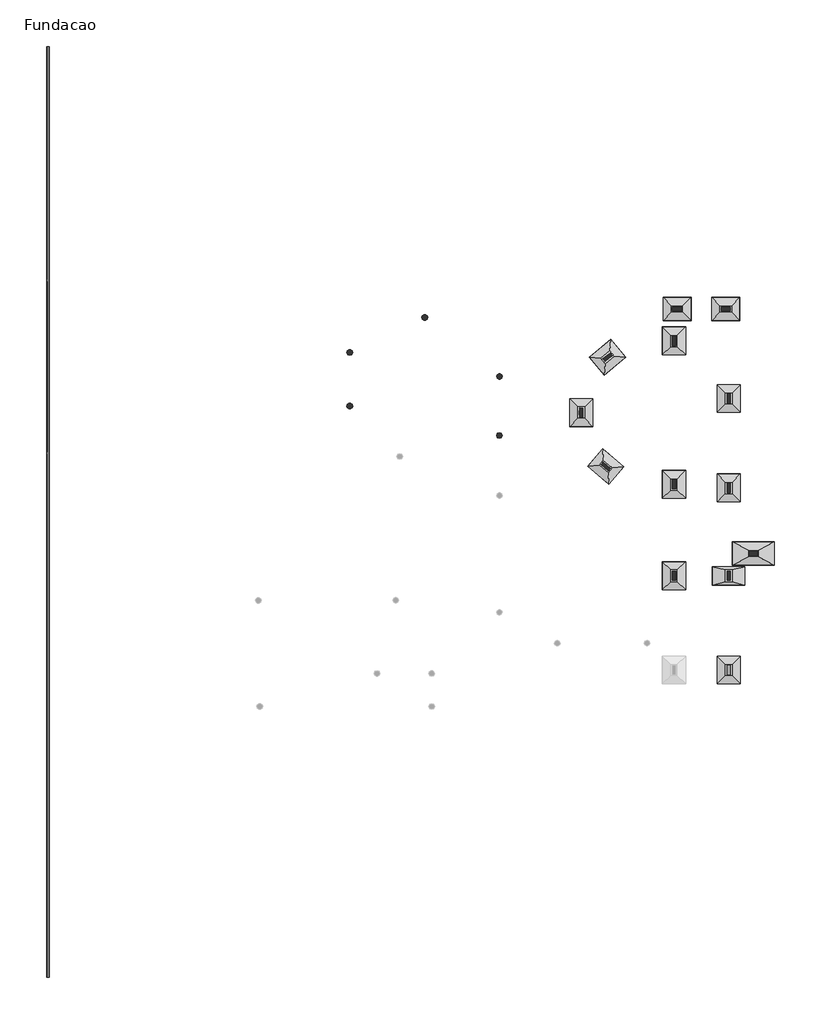
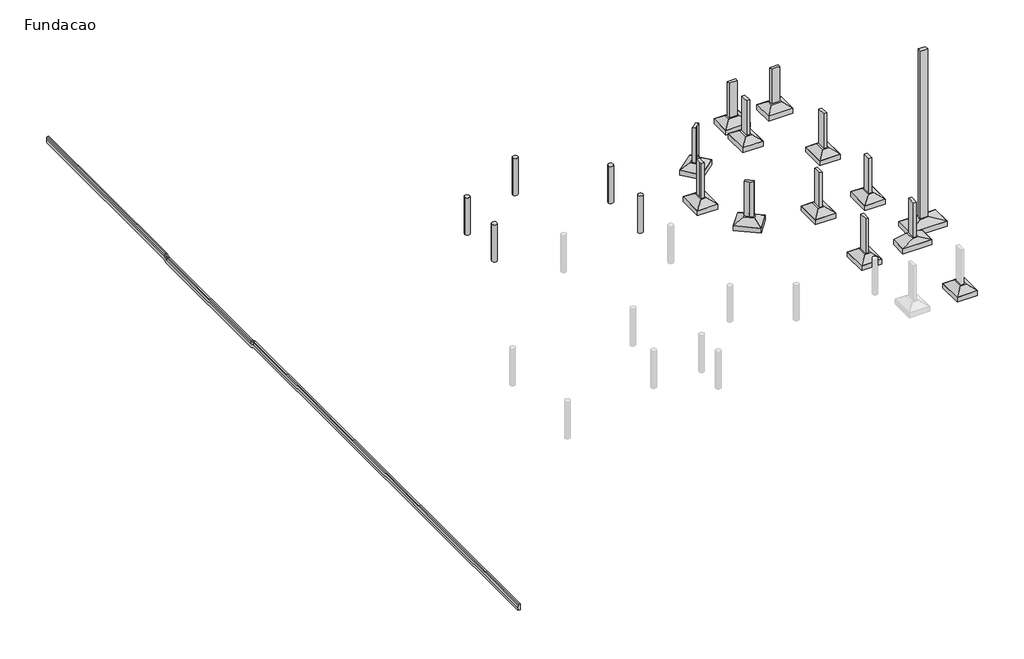
# One storey, part 2 of 2: 17 columns, 13 fasteners, 1 proxy.
# Revit data of these elements (continued)
# Element 2 (IfcColumn, "TQS - Pilar circular : TQS - Pilar circular 25.0cm") (continued)
#   Pino = ""
#   Distribuicao = ""
#   Solidarizado = ""
#   Solidarizar na montagem = ""
#   Unir com o próximo = ""
#   Grupo pre moldado = ""
#   Verificado = ""
#   Concreto C = ""
#   Taxa de armadura (kgf/m³) = 0
#   Carga (tf/m²) = 0
#   Carga (tf/m) = 0
#   Carga (tf) = 0
#   Altura = 1.70 m
#   Rebaixo = 0.00 m
#   Altura da fundacao = 0.00 m
#   Largura = 0.00 m
#   Distancia a face = 0.00 m
#   Distancia ao eixo = 0.00 m
#   Resultado de Ensaios fck (MPa) = 0
#   Unique TQS ID = -766
#   Principal = yes
#   Nasce = yes
#   Morre = yes
#   Cabeca de Pilar = no
#   Structural Material = Concrete - Cast-in-Place Concrete
#   Phase Created = CC_PE
#   Materials on its faces: "Concrete - Cast-in-Place Concrete"
# Element 3 (IfcColumn, "TQS - Pilar circular : TQS - Pilar circular 25.0cm")
#   Uso = "ESTRUTURA"
#   Titulo = "B5"
#   Chave = "B5//0"
#   Tipo Elemento = "Pilar"
#   SHA1 = "B6B3AE0C1195346A87609D6969D28A00933EE0AE"
#   Revisão = ""
#   Tipo de carga = ""
#   Divisor de flexao = ""
#   Secao = "C 25"
#   Configuracao = ""
#   Angulo (graus) = ""
#   Detalhamento = ""
#   Casos de vento manual = ""
#   Tipo = ""
#   Alcas = ""
#   Furos = ""
#   Pino = ""
#   Distribuicao = ""
#   Solidarizado = ""
#   Solidarizar na montagem = ""
#   Unir com o próximo = ""
#   Grupo pre moldado = ""
#   Verificado = ""
#   Concreto C = ""
#   Taxa de armadura (kgf/m³) = 0
#   Carga (tf/m²) = 0
#   Carga (tf/m) = 0
#   Carga (tf) = 0
#   Altura = 1.70 m
#   Rebaixo = 0.00 m
#   Altura da fundacao = 0.00 m
#   Largura = 0.00 m
#   Distancia a face = 0.00 m
#   Distancia ao eixo = 0.00 m
#   Resultado de Ensaios fck (MPa) = 0
#   Unique TQS ID = -767
#   Principal = yes
#   Nasce = yes
#   Morre = yes
#   Cabeca de Pilar = no
#   Structural Material = Concrete - Cast-in-Place Concrete
#   Phase Created = CC_PE
#   Materials on its faces: "Concrete - Cast-in-Place Concrete"
# Element 4 (IfcColumn, "TQS - Pilar circular : TQS - Pilar circular 25.0cm")
#   Uso = "ESTRUTURA"
#   Titulo = "B3"
#   Chave = "B3//0"
#   Tipo Elemento = "Pilar"
#   SHA1 = "B4824BA6EB04DBA88013BAD919A11F987E93A8CE"
#   Revisão = ""
#   Tipo de carga = ""
#   Divisor de flexao = ""
#   Secao = "C 25"
#   Configuracao = ""
#   Angulo (graus) = ""
#   Detalhamento = ""
#   Casos de vento manual = ""
#   Tipo = ""
#   Alcas = ""
#   Furos = ""
#   Pino = ""
#   Distribuicao = ""
#   Solidarizado = ""
#   Solidarizar na montagem = ""
#   Unir com o próximo = ""
#   Grupo pre moldado = ""
#   Verificado = ""
#   Concreto C = ""
#   Taxa de armadura (kgf/m³) = 0
#   Carga (tf/m²) = 0
#   Carga (tf/m) = 0
#   Carga (tf) = 0
#   Altura = 1.70 m
#   Rebaixo = 0.00 m
#   Altura da fundacao = 0.00 m
#   Largura = 0.00 m
#   Distancia a face = 0.00 m
#   Distancia ao eixo = 0.00 m
#   Resultado de Ensaios fck (MPa) = 0
#   Unique TQS ID = -768
#   Principal = yes
#   Nasce = yes
#   Morre = yes
#   Cabeca de Pilar = no
#   Structural Material = Concrete - Cast-in-Place Concrete
#   Phase Created = CC_PE
#   Materials on its faces: "Concrete - Cast-in-Place Concrete"
# Element 5 (IfcColumn, "TQS - Pilar circular : TQS - Pilar circular 25.0cm")
#   Uso = "ESTRUTURA"
#   Titulo = "B2"
#   Chave = "B2//0"
#   Tipo Elemento = "Pilar"
#   SHA1 = "4CE2E912DC9B0318D735B89447CA6954BE93FBBD"
#   Revisão = ""
#   Tipo de carga = ""
#   Divisor de flexao = ""
#   Secao = "C 25"
#   Configuracao = ""
#   Angulo (graus) = ""
#   Detalhamento = ""
#   Casos de vento manual = ""
#   Tipo = ""
#   Alcas = ""
#   Furos = ""
#   Pino = ""
#   Distribuicao = ""
#   Solidarizado = ""
#   Solidarizar na montagem = ""
#   Unir com o próximo = ""
#   Grupo pre moldado = ""
#   Verificado = ""
#   Concreto C = ""
#   Taxa de armadura (kgf/m³) = 0
#   Carga (tf/m²) = 0
#   Carga (tf/m) = 0
#   Carga (tf) = 0
#   Altura = 1.70 m
#   Rebaixo = 0.00 m
#   Altura da fundacao = 0.00 m
#   Largura = 0.00 m
#   Distancia a face = 0.00 m
#   Distancia ao eixo = 0.00 m
#   Resultado de Ensaios fck (MPa) = 0
#   Unique TQS ID = -773
#   Principal = yes
#   Nasce = yes
#   Morre = yes
#   Cabeca de Pilar = no
#   Structural Material = Concrete - Cast-in-Place Concrete
#   Phase Created = CC_PE
#   Materials on its faces: "Concrete - Cast-in-Place Concrete"
# Element 6 (IfcColumn, "TQS - Pilar circular : TQS - Pilar circular 25.0cm")
#   Uso = "ESTRUTURA"
#   Titulo = "B4"
#   Chave = "B4//0"
#   Tipo Elemento = "Pilar"
#   SHA1 = "33C063B82A35DA14032FDD3FDBBCC7600ACCE04D"
#   Revisão = ""
#   Tipo de carga = ""
#   Divisor de flexao = ""
#   Secao = "C 25"
#   Configuracao = ""
#   Angulo (graus) = ""
#   Detalhamento = ""
#   Casos de vento manual = ""
#   Tipo = ""
#   Alcas = ""
#   Furos = ""
#   Pino = ""
#   Distribuicao = ""
#   Solidarizado = ""
#   Solidarizar na montagem = ""
#   Unir com o próximo = ""
#   Grupo pre moldado = ""
#   Verificado = ""
#   Concreto C = ""
#   Taxa de armadura (kgf/m³) = 0
#   Carga (tf/m²) = 0
#   Carga (tf/m) = 0
#   Carga (tf) = 0
#   Altura = 1.70 m
#   Rebaixo = 0.00 m
#   Altura da fundacao = 0.00 m
#   Largura = 0.00 m
#   Distancia a face = 0.00 m
#   Distancia ao eixo = 0.00 m
#   Resultado de Ensaios fck (MPa) = 0
#   Unique TQS ID = -774
#   Principal = yes
#   Nasce = yes
#   Morre = yes
#   Cabeca de Pilar = no
#   Structural Material = Concrete - Cast-in-Place Concrete
#   Phase Created = CC_PE
#   Materials on its faces: "Concrete - Cast-in-Place Concrete"
# Element 7 (IfcColumn, "TQS - Pilar retangular : 14.0 x 40.0")
#   Uso = "ESTRUTURA"
#   Titulo = "PS1"
#   Chave = "PS1//0"
#   Tipo Elemento = "Pilar"
#   SHA1 = "4597F8CE5B5008DD3216867DEF2D1334C590FC15"
#   Revisão = ""
#   Tipo de carga = ""
#   Divisor de flexao = ""
#   Secao = "R 14/40 270°"
#   Configuracao = ""
#   Angulo (graus) = ""
#   Detalhamento = ""
#   Casos de vento manual = ""
#   Tipo = ""
#   Alcas = ""
#   Furos = ""
#   Pino = ""
#   Distribuicao = ""
#   Solidarizado = ""
#   Solidarizar na montagem = ""
#   Unir com o próximo = ""
#   Grupo pre moldado = ""
#   Verificado = ""
#   Concreto C = ""
#   Taxa de armadura (kgf/m³) = 0
#   Carga (tf/m²) = 0
#   Carga (tf/m) = 0
#   Carga (tf) = 0
#   Altura = 1.70 m
#   Rebaixo = 0.00 m
#   Altura da fundacao = 0.00 m
#   Largura = 0.00 m
#   Distancia a face = 0.00 m
#   Distancia ao eixo = 0.00 m
#   Resultado de Ensaios fck (MPa) = 0
#   Unique TQS ID = -958
#   Principal = yes
#   Nasce = yes
#   Morre = yes
#   Cabeca de Pilar = no
#   Structural Material = Concrete - Cast-in-Place Concrete
#   Phase Created = CC_PE
#   Materials on its faces: "Concrete - Cast-in-Place Concrete"
# Element 8 (IfcColumn, "TQS - Pilar retangular : 14.0 x 40.0")
#   Uso = "ESTRUTURA"
#   Titulo = "PS2"
#   Chave = "PS2//0"
#   Tipo Elemento = "Pilar"
#   SHA1 = "1729CD9DA72122FACD843418D908847D3B1966CD"
#   Revisão = ""
#   Tipo de carga = ""
#   Divisor de flexao = ""
#   Secao = "R 14/40 270°"
#   Configuracao = ""
#   Angulo (graus) = ""
#   Detalhamento = ""
#   Casos de vento manual = ""
#   Tipo = ""
#   Alcas = ""
#   Furos = ""
#   Pino = ""
#   Distribuicao = ""
#   Solidarizado = ""
#   Solidarizar na montagem = ""
#   Unir com o próximo = ""
#   Grupo pre moldado = ""
#   Verificado = ""
#   Concreto C = ""
#   Taxa de armadura (kgf/m³) = 0
#   Carga (tf/m²) = 0
#   Carga (tf/m) = 0
#   Carga (tf) = 0
#   Altura = 1.70 m
#   Rebaixo = 0.00 m
#   Altura da fundacao = 0.00 m
#   Largura = 0.00 m
#   Distancia a face = 0.00 m
#   Distancia ao eixo = 0.00 m
#   Resultado de Ensaios fck (MPa) = 0
#   Unique TQS ID = -959
#   Principal = yes
#   Nasce = yes
#   Morre = yes
#   Cabeca de Pilar = no
#   Structural Material = Concrete - Cast-in-Place Concrete
#   Phase Created = CC_PE
#   Materials on its faces: "Concrete - Cast-in-Place Concrete"
# Element 9 (IfcColumn, "TQS - Pilar retangular : 14.0 x 40.0")
#   Uso = "ESTRUTURA"
#   Titulo = "PS3"
#   Chave = "PS3//0"
#   Tipo Elemento = "Pilar"
#   SHA1 = "E1C4E1DD2B85E2F78CE9D8770BC24705A0EC4463"
#   Revisão = ""
#   Tipo de carga = ""
#   Divisor de flexao = ""
#   Secao = "R 14/40 180°"
#   Configuracao = ""
#   Angulo (graus) = ""
#   Detalhamento = ""
#   Casos de vento manual = ""
#   Tipo = ""
#   Alcas = ""
#   Furos = ""
#   Pino = ""
#   Distribuicao = ""
#   Solidarizado = ""
#   Solidarizar na montagem = ""
#   Unir com o próximo = ""
#   Grupo pre moldado = ""
#   Verificado = ""
#   Concreto C = ""
#   Taxa de armadura (kgf/m³) = 0
#   Carga (tf/m²) = 0
#   Carga (tf/m) = 0
#   Carga (tf) = 0
#   Altura = 1.70 m
#   Rebaixo = 0.00 m
#   Altura da fundacao = 0.00 m
#   Largura = 0.00 m
#   Distancia a face = 0.00 m
#   Distancia ao eixo = 0.00 m
#   Resultado de Ensaios fck (MPa) = 0
#   Unique TQS ID = -960
#   Principal = yes
#   Nasce = yes
#   Morre = yes
#   Cabeca de Pilar = no
#   Structural Material = Concrete - Cast-in-Place Concrete
#   Phase Created = CC_PE
#   Materials on its faces: "Concrete - Cast-in-Place Concrete"
# Element 10 (IfcColumn, "TQS - Pilar retangular : 14.0 x 40.0")
#   Uso = "ESTRUTURA"
#   Titulo = "PS7"
#   Chave = "PS7//0"
#   Tipo Elemento = "Pilar"
#   SHA1 = "EE51B7F018C373FE9CEF53A9864C8051348A9FB9"
#   Revisão = ""
#   Tipo de carga = ""
#   Divisor de flexao = ""
#   Secao = "R 14/40 180°"
#   Configuracao = ""
#   Angulo (graus) = ""
#   Detalhamento = ""
#   Casos de vento manual = ""
#   Tipo = ""
#   Alcas = ""
#   Furos = ""
#   Pino = ""
#   Distribuicao = ""
#   Solidarizado = ""
#   Solidarizar na montagem = ""
#   Unir com o próximo = ""
#   Grupo pre moldado = ""
#   Verificado = ""
#   Concreto C = ""
#   Taxa de armadura (kgf/m³) = 0
#   Carga (tf/m²) = 0
#   Carga (tf/m) = 0
#   Carga (tf) = 0
#   Altura = 1.70 m
#   Rebaixo = 0.00 m
#   Altura da fundacao = 0.00 m
#   Largura = 0.00 m
#   Distancia a face = 0.00 m
#   Distancia ao eixo = 0.00 m
#   Resultado de Ensaios fck (MPa) = 0
#   Unique TQS ID = -964
#   Principal = yes
#   Nasce = yes
#   Morre = yes
#   Cabeca de Pilar = no
#   Structural Material = Concrete - Cast-in-Place Concrete
#   Phase Created = CC_PE
#   Materials on its faces: "Concrete - Cast-in-Place Concrete"
# Element 11 (IfcColumn, "TQS - Pilar retangular : 14.0 x 40.0")
#   Uso = "ESTRUTURA"
#   Titulo = "PS8"
#   Chave = "PS8//0"
#   Tipo Elemento = "Pilar"
#   SHA1 = "B515A8CC25CBD0A114828B82A1075E16319BC015"
#   Revisão = ""
#   Tipo de carga = ""
#   Divisor de flexao = ""
#   Secao = "R 14/40 180°"
#   Configuracao = ""
#   Angulo (graus) = ""
#   Detalhamento = ""
#   Casos de vento manual = ""
#   Tipo = ""
#   Alcas = ""
#   Furos = ""
#   Pino = ""
#   Distribuicao = ""
#   Solidarizado = ""
#   Solidarizar na montagem = ""
#   Unir com o próximo = ""
#   Grupo pre moldado = ""
#   Verificado = ""
#   Concreto C = ""
#   Taxa de armadura (kgf/m³) = 0
#   Carga (tf/m²) = 0
#   Carga (tf/m) = 0
#   Carga (tf) = 0
#   Altura = 1.70 m
#   Rebaixo = 0.00 m
#   Altura da fundacao = 0.00 m
#   Largura = 0.00 m
#   Distancia a face = 0.00 m
#   Distancia ao eixo = 0.00 m
#   Resultado de Ensaios fck (MPa) = 0
#   Unique TQS ID = -965
#   Principal = yes
#   Nasce = yes
#   Morre = yes
#   Cabeca de Pilar = no
#   Structural Material = Concrete - Cast-in-Place Concrete
#   Phase Created = CC_PE
#   Materials on its faces: "Concrete - Cast-in-Place Concrete"
# Element 12 (IfcColumn, "TQS - Pilar retangular : 14.0 x 40.0")
#   Uso = "ESTRUTURA"
#   Titulo = "PS11"
#   Chave = "PS11//0"
#   Tipo Elemento = "Pilar"
#   SHA1 = "38C3E9E25C80C043D595FE86FE1A911FDC38D350"
#   Revisão = ""
#   Tipo de carga = ""
#   Divisor de flexao = ""
#   Secao = "R 14/40 180°"
#   Configuracao = ""
#   Angulo (graus) = ""
#   Detalhamento = ""
#   Casos de vento manual = ""
#   Tipo = ""
#   Alcas = ""
#   Furos = ""
#   Pino = ""
#   Distribuicao = ""
#   Solidarizado = ""
#   Solidarizar na montagem = ""
#   Unir com o próximo = ""
#   Grupo pre moldado = ""
#   Verificado = ""
#   Concreto C = ""
#   Taxa de armadura (kgf/m³) = 0
#   Carga (tf/m²) = 0
#   Carga (tf/m) = 0
#   Carga (tf) = 0
#   Altura = 1.70 m
#   Rebaixo = 0.00 m
#   Altura da fundacao = 0.00 m
#   Largura = 0.00 m
#   Distancia a face = 0.00 m
#   Distancia ao eixo = 0.00 m
#   Resultado de Ensaios fck (MPa) = 0
#   Unique TQS ID = -968
#   Principal = yes
#   Nasce = yes
#   Morre = yes
#   Cabeca de Pilar = no
#   Structural Material = Concrete - Cast-in-Place Concrete
#   Phase Created = CC_PE
#   Materials on its faces: "Concrete - Cast-in-Place Concrete"
# Element 13 (IfcColumn, "TQS - Pilar retangular : 14.0 x 40.0")
#   Uso = "ESTRUTURA"
#   Titulo = "PS12"
#   Chave = "PS12//0"
#   Tipo Elemento = "Pilar"
#   SHA1 = "512D0DE7DB718BC0FE0AECE12A9FB23F7FBE26A9"
#   Revisão = ""
#   Tipo de carga = ""
#   Divisor de flexao = ""
#   Secao = "R 14/40 180°"
#   Configuracao = ""
#   Angulo (graus) = ""
#   Detalhamento = ""
#   Casos de vento manual = ""
#   Tipo = ""
#   Alcas = ""
#   Furos = ""
#   Pino = ""
#   Distribuicao = ""
#   Solidarizado = ""
#   Solidarizar na montagem = ""
#   Unir com o próximo = ""
#   Grupo pre moldado = ""
#   Verificado = ""
#   Concreto C = ""
#   Taxa de armadura (kgf/m³) = 0
#   Carga (tf/m²) = 0
#   Carga (tf/m) = 0
#   Carga (tf) = 0
#   Altura = 1.70 m
#   Rebaixo = 0.00 m
#   Altura da fundacao = 0.00 m
#   Largura = 0.00 m
#   Distancia a face = 0.00 m
#   Distancia ao eixo = 0.00 m
#   Resultado de Ensaios fck (MPa) = 0
#   Unique TQS ID = -969
#   Principal = yes
#   Nasce = yes
#   Morre = yes
#   Cabeca de Pilar = no
#   Structural Material = Concrete - Cast-in-Place Concrete
#   Phase Created = CC_PE
#   Materials on its faces: "Concrete - Cast-in-Place Concrete"
# Element 14 (IfcColumn, "TQS - Pilar retangular : 14.0 x 40.0")
#   Uso = "ESTRUTURA"
#   Titulo = "PS13"
#   Chave = "PS13//0"
#   Tipo Elemento = "Pilar"
#   SHA1 = "8EC8E2C6B90DD4DF760F1D4ED431316ED84D10F2"
#   Revisão = ""
#   Tipo de carga = ""
#   Divisor de flexao = ""
#   Secao = "R 14/40 180°"
#   Configuracao = ""
#   Angulo (graus) = ""
#   Detalhamento = ""
#   Casos de vento manual = ""
#   Tipo = ""
#   Alcas = ""
#   Furos = ""
#   Pino = ""
#   Distribuicao = ""
#   Solidarizado = ""
#   Solidarizar na montagem = ""
#   Unir com o próximo = ""
#   Grupo pre moldado = ""
#   Verificado = ""
#   Concreto C = ""
#   Taxa de armadura (kgf/m³) = 0
#   Carga (tf/m²) = 0
#   Carga (tf/m) = 0
#   Carga (tf) = 0
#   Altura = 1.70 m
#   Rebaixo = 0.00 m
#   Altura da fundacao = 0.00 m
#   Largura = 0.00 m
#   Distancia a face = 0.00 m
#   Distancia ao eixo = 0.00 m
#   Resultado de Ensaios fck (MPa) = 0
#   Unique TQS ID = -970
#   Principal = yes
#   Nasce = yes
#   Morre = yes
#   Cabeca de Pilar = no
#   Structural Material = Concrete - Cast-in-Place Concrete
#   Phase Created = CC_PE
#   Materials on its faces: "Concrete - Cast-in-Place Concrete"
# Element 15 (IfcColumn, "TQS - Pilar retangular : 19.0 x 35.0")
#   Uso = "ESTRUTURA"
#   Titulo = "P14"
#   Chave = "P14//0"
#   Tipo Elemento = "Pilar"
#   SHA1 = "6631C03D899D7914EBA5EACF44BE1498A45C603B"
#   Revisão = ""
#   Tipo de carga = ""
#   Divisor de flexao = ""
#   Secao = "R 19/35 90°"
#   Configuracao = ""
#   Angulo (graus) = ""
#   Detalhamento = ""
#   Casos de vento manual = ""
#   Tipo = ""
#   Alcas = ""
#   Furos = ""
#   Pino = ""
#   Distribuicao = ""
#   Solidarizado = ""
#   Solidarizar na montagem = ""
#   Unir com o próximo = ""
#   Grupo pre moldado = ""
#   Verificado = ""
#   Concreto C = ""
#   Taxa de armadura (kgf/m³) = 0
#   Carga (tf/m²) = 0
#   Carga (tf/m) = 0
#   Carga (tf) = 0
#   Altura = 7.85 m
#   Rebaixo = 0.00 m
#   Altura da fundacao = 0.00 m
#   Largura = 0.00 m
#   Distancia a face = 0.00 m
#   Distancia ao eixo = 0.00 m
#   Resultado de Ensaios fck (MPa) = 0
#   Unique TQS ID = -30
#   Principal = yes
#   Nasce = yes
#   Morre = yes
#   Cabeca de Pilar = no
#   Structural Material = Concrete - Cast-in-Place Concrete
#   Phase Created = CC_PE
#   Materials on its faces: "Concrete - Cast-in-Place Concrete"
# Element 16 (IfcColumn, "TQS - Pilar Polig_1 : TQS Column")
#   Uso = "ESTRUTURA"
#   Titulo = "PS4"
#   Chave = "PS4//0"
#   Tipo Elemento = "Pilar"
#   SHA1 = "CAF5758E71A5FE097847EBD6542E0EE23CE53B7B"
#   Revisão = ""
#   Tipo de carga = ""
#   Divisor de flexao = ""
#   Secao = "P  - Poligonal"
#   Configuracao = ""
#   Angulo (graus) = ""
#   Detalhamento = ""
#   Casos de vento manual = ""
#   Tipo = ""
#   Alcas = ""
#   Furos = ""
#   Pino = ""
#   Distribuicao = ""
#   Solidarizado = ""
#   Solidarizar na montagem = ""
#   Unir com o próximo = ""
#   Grupo pre moldado = ""
#   Verificado = ""
#   Concreto C = ""
#   Taxa de armadura (kgf/m³) = 0
#   Carga (tf/m²) = 0
#   Carga (tf/m) = 0
#   Carga (tf) = 0
#   Altura = 1.70 m
#   Rebaixo = 0.00 m
#   Altura da fundacao = 0.00 m
#   Largura = 0.00 m
#   Distancia a face = 0.00 m
#   Distancia ao eixo = 0.00 m
#   Resultado de Ensaios fck (MPa) = 0
#   Unique TQS ID = -961
#   Principal = yes
#   Nasce = yes
#   Morre = yes
#   Cabeca de Pilar = no
#   Structural Material = Concrete - Cast-in-Place Concrete
#   Phase Created = CC_PE
# Element 17 (IfcColumn, "TQS - Pilar Polig_1 : TQS Column")
#   Uso = "ESTRUTURA"
#   Titulo = "PS5"
#   Chave = "PS5//0"
#   Tipo Elemento = "Pilar"
#   SHA1 = "AE9BDBDC0B1786B9555B7E0CE4AAD4E849800AD1"
#   Revisão = ""
#   Tipo de carga = ""
#   Divisor de flexao = ""
#   Secao = "P  - Poligonal"
#   Configuracao = ""
#   Angulo (graus) = ""
#   Detalhamento = ""
#   Casos de vento manual = ""
#   Tipo = ""
#   Alcas = ""
#   Furos = ""
#   Pino = ""
#   Distribuicao = ""
#   Solidarizado = ""
#   Solidarizar na montagem = ""
#   Unir com o próximo = ""
#   Grupo pre moldado = ""
#   Verificado = ""
#   Concreto C = ""
#   Taxa de armadura (kgf/m³) = 0
#   Carga (tf/m²) = 0
#   Carga (tf/m) = 0
#   Carga (tf) = 0
#   Altura = 1.70 m
#   Rebaixo = 0.00 m
#   Altura da fundacao = 0.00 m
#   Largura = 0.00 m
#   Distancia a face = 0.00 m
#   Distancia ao eixo = 0.00 m
#   Resultado de Ensaios fck (MPa) = 0
#   Unique TQS ID = -962
#   Principal = yes
#   Nasce = yes
#   Morre = yes
#   Cabeca de Pilar = no
#   Structural Material = Concrete - Cast-in-Place Concrete
#   Phase Created = CC_PE
# Element 18 (IfcColumn, "TQS - Pilar Polig_2 : TQS Column")
#   Uso = "ESTRUTURA"
#   Titulo = "PS6"
#   Chave = "PS6//0"
#   Tipo Elemento = "Pilar"
#   SHA1 = "07EEAEB0E5A3D9C7C5812BCB6FDA506A68E4D4F2"
#   Revisão = ""
#   Tipo de carga = ""
#   Divisor de flexao = ""
#   Secao = "P  - Poligonal"
#   Configuracao = ""
#   Angulo (graus) = ""
#   Detalhamento = ""
#   Casos de vento manual = ""
#   Tipo = ""
#   Alcas = ""
#   Furos = ""
#   Pino = ""
#   Distribuicao = ""
#   Solidarizado = ""
#   Solidarizar na montagem = ""
#   Unir com o próximo = ""
#   Grupo pre moldado = ""
#   Verificado = ""
#   Concreto C = ""
#   Taxa de armadura (kgf/m³) = 0
#   Carga (tf/m²) = 0
#   Carga (tf/m) = 0
#   Carga (tf) = 0
#   Altura = 1.70 m
#   Rebaixo = 0.00 m
#   Altura da fundacao = 0.00 m
#   Largura = 0.00 m
#   Distancia a face = 0.00 m
#   Distancia ao eixo = 0.00 m
#   Resultado de Ensaios fck (MPa) = 0
#   Unique TQS ID = -963
#   Principal = yes
#   Nasce = yes
#   Morre = yes
#   Cabeca de Pilar = no
#   Structural Material = Concrete - Cast-in-Place Concrete
#   Phase Created = CC_PE
# Element 19 (IfcFastener, "TQS - Sapata : S14")
#   Uso = "ESTRUTURA"
#   Titulo = "S14"
#   Chave = "-1550"
#   Tipo Elemento = "Fundação"
#   SHA1 = "1357E856F80250D7EFC9EC1E050D5963CC884844"
#   Revisão = ""
#   Tipo de carga = ""
#   Divisor de flexao = ""
#   Secao = ""
#   Configuracao = ""
#   Angulo (graus) = ""
#   Detalhamento = ""
#   Casos de vento manual = ""
#   Tipo = "Sapata"
#   Dimensoes = "100.0,180.0"
#   Estacas = ""
#   Calice = ""
#   Rugosidade = ""
#   Alcas = ""
#   Furos = ""
#   Pino = ""
#   Distribuicao = ""
#   Solidarizado = ""
#   Solidarizar na montagem = ""
#   Unir com o próximo = ""
#   Grupo pre moldado = ""
#   Verificado = ""
#   Concreto C = ""
#   Taxa de armadura (kgf/m³) = 0
#   Carga (tf/m²) = 0
#   Carga (tf/m) = 0
#   Carga (tf) = 0
#   Altura = 0.00 m
#   Rebaixo = 0.00 m
#   Pilar ficticio = 0.00 m
#   Topo = -1.45 m
#   Altura total = 0.50 m
#   Rodape = 0.00 m
#   Diametro = 0.00 m
#   Altura dentro do bloco = 0.00 m
#   Entre eixos = 0.00 m
#   Paredes = 0.00 m
#   Caimento = 0.00 m
#   Largura = 0.00 m
#   Distancia a face = 0.00 m
#   Distancia ao eixo = 0.00 m
#   Resultado de Ensaios fck (MPa) = 0
#   Unique TQS ID = -1550
#   Principal = yes
#   Phase Created = CC_PE
#   Materials on its faces: "Concreto - Concreto concretado no local"
# Element 20 (IfcFastener, "TQS - Sapata : SPS1")
#   Uso = "ESTRUTURA"
#   Titulo = "SPS1"
#   Chave = "-1512"
#   Tipo Elemento = "Fundação"
#   SHA1 = "0DB0C78ACFE2E409544A77F7853F60381CB93818"
#   Revisão = ""
#   Tipo de carga = ""
#   Divisor de flexao = ""
#   Secao = ""
#   Configuracao = ""
#   Angulo (graus) = ""
#   Detalhamento = ""
#   Casos de vento manual = ""
#   Tipo = "Sapata"
#   Dimensoes = "100.0,120.0"
#   Estacas = ""
#   Calice = ""
#   Rugosidade = ""
#   Alcas = ""
#   Furos = ""
#   Pino = ""
#   Distribuicao = ""
#   Solidarizado = ""
#   Solidarizar na montagem = ""
#   Unir com o próximo = ""
#   Grupo pre moldado = ""
#   Verificado = ""
#   Concreto C = ""
#   Taxa de armadura (kgf/m³) = 0
#   Carga (tf/m²) = 0
#   Carga (tf/m) = 0
#   Carga (tf) = 0
#   Altura = 0.00 m
#   Rebaixo = 0.00 m
#   Pilar ficticio = 0.00 m
#   Topo = -1.45 m
#   Altura total = 0.50 m
#   Rodape = 0.00 m
#   Diametro = 0.00 m
#   Altura dentro do bloco = 0.00 m
#   Entre eixos = 0.00 m
#   Paredes = 0.00 m
#   Caimento = 0.00 m
#   Largura = 0.00 m
#   Distancia a face = 0.00 m
#   Distancia ao eixo = 0.00 m
#   Resultado de Ensaios fck (MPa) = 0
#   Unique TQS ID = -1512
#   Principal = yes
#   Phase Created = CC_PE
#   Materials on its faces: "Concreto - Concreto concretado no local"
# Element 21 (IfcFastener, "TQS - Sapata : SPS10")
#   Uso = "ESTRUTURA"
#   Titulo = "SPS10"
#   Chave = "-1543"
#   Tipo Elemento = "Fundação"
#   SHA1 = "612F949682BC8906AE43999ACE3B00A4C616A0A8"
#   Revisão = ""
#   Tipo de carga = ""
#   Divisor de flexao = ""
#   Secao = ""
#   Configuracao = ""
#   Angulo (graus) = ""
#   Detalhamento = ""
#   Casos de vento manual = ""
#   Tipo = "Sapata"
#   Dimensoes = "100.0,120.0"
#   Estacas = ""
#   Calice = ""
#   Rugosidade = ""
#   Alcas = ""
#   Furos = ""
#   Pino = ""
#   Distribuicao = ""
#   Solidarizado = ""
#   Solidarizar na montagem = ""
#   Unir com o próximo = ""
#   Grupo pre moldado = ""
#   Verificado = ""
#   Concreto C = ""
#   Taxa de armadura (kgf/m³) = 0
#   Carga (tf/m²) = 0
#   Carga (tf/m) = 0
#   Carga (tf) = 0
#   Altura = 0.00 m
#   Rebaixo = 0.00 m
#   Pilar ficticio = 0.00 m
#   Topo = -1.45 m
#   Altura total = 0.50 m
#   Rodape = 0.00 m
#   Diametro = 0.00 m
#   Altura dentro do bloco = 0.00 m
#   Entre eixos = 0.00 m
#   Paredes = 0.00 m
#   Caimento = 0.00 m
#   Largura = 0.00 m
#   Distancia a face = 0.00 m
#   Distancia ao eixo = 0.00 m
#   Resultado de Ensaios fck (MPa) = 0
#   Unique TQS ID = -1543
#   Principal = yes
#   Phase Created = CC_PE
#   Materials on its faces: "Concreto - Concreto concretado no local"
# Element 22 (IfcFastener, "TQS - Sapata : SPS11")
#   Uso = "ESTRUTURA"
#   Titulo = "SPS11"
#   Chave = "-1544"
#   Tipo Elemento = "Fundação"
#   SHA1 = "678A094029D3186700C53CC9859E21CCB03EEAB8"
#   Revisão = ""
#   Tipo de carga = ""
#   Divisor de flexao = ""
#   Secao = ""
#   Configuracao = ""
#   Angulo (graus) = ""
#   Detalhamento = ""
#   Casos de vento manual = ""
#   Tipo = "Sapata"
#   Dimensoes = "140.0,80.0"
#   Estacas = ""
#   Calice = ""
#   Rugosidade = ""
#   Alcas = ""
#   Furos = ""
#   Pino = ""
#   Distribuicao = ""
#   Solidarizado = ""
#   Solidarizar na montagem = ""
#   Unir com o próximo = ""
#   Grupo pre moldado = ""
#   Verificado = ""
#   Concreto C = ""
#   Taxa de armadura (kgf/m³) = 0
#   Carga (tf/m²) = 0
#   Carga (tf/m) = 0
#   Carga (tf) = 0
#   Altura = 0.00 m
#   Rebaixo = 0.00 m
#   Pilar ficticio = 0.00 m
#   Topo = -1.45 m
#   Altura total = 0.50 m
#   Rodape = 0.00 m
#   Diametro = 0.00 m
#   Altura dentro do bloco = 0.00 m
#   Entre eixos = 0.00 m
#   Paredes = 0.00 m
#   Caimento = 0.00 m
#   Largura = 0.00 m
#   Distancia a face = 0.00 m
#   Distancia ao eixo = 0.00 m
#   Resultado de Ensaios fck (MPa) = 0
#   Unique TQS ID = -1544
#   Principal = yes
#   Phase Created = CC_PE
#   Materials on its faces: "Concreto - Concreto concretado no local"
# Element 23 (IfcFastener, "TQS - Sapata : SPS12")
#   Uso = "ESTRUTURA"
#   Titulo = "SPS12"
#   Chave = "-1545"
#   Tipo Elemento = "Fundação"
#   SHA1 = "A892B9C9285BE3407F8B32028442AB264075CE3A"
#   Revisão = ""
#   Tipo de carga = ""
#   Divisor de flexao = ""
#   Secao = ""
#   Configuracao = ""
#   Angulo (graus) = ""
#   Detalhamento = ""
#   Casos de vento manual = ""
#   Tipo = "Sapata"
#   Dimensoes = "100.0,120.0"
#   Estacas = ""
#   Calice = ""
#   Rugosidade = ""
#   Alcas = ""
#   Furos = ""
#   Pino = ""
#   Distribuicao = ""
#   Solidarizado = ""
#   Solidarizar na montagem = ""
#   Unir com o próximo = ""
#   Grupo pre moldado = ""
#   Verificado = ""
#   Concreto C = ""
#   Taxa de armadura (kgf/m³) = 0
#   Carga (tf/m²) = 0
#   Carga (tf/m) = 0
#   Carga (tf) = 0
#   Altura = 0.00 m
#   Rebaixo = 0.00 m
#   Pilar ficticio = 0.00 m
#   Topo = -1.45 m
#   Altura total = 0.50 m
#   Rodape = 0.00 m
#   Diametro = 0.00 m
#   Altura dentro do bloco = 0.00 m
#   Entre eixos = 0.00 m
#   Paredes = 0.00 m
#   Caimento = 0.00 m
#   Largura = 0.00 m
#   Distancia a face = 0.00 m
#   Distancia ao eixo = 0.00 m
#   Resultado de Ensaios fck (MPa) = 0
#   Unique TQS ID = -1545
#   Principal = yes
#   Phase Created = CC_PE
#   Materials on its faces: "Concreto - Concreto concretado no local"
# Element 24 (IfcFastener, "TQS - Sapata : SPS13")
#   Uso = "ESTRUTURA"
#   Titulo = "SPS13"
#   Chave = "-1546"
#   Tipo Elemento = "Fundação"
#   SHA1 = "CDD7149D511DCC0D87C76189E976442BBC013FA0"
#   Revisão = ""
#   Tipo de carga = ""
#   Divisor de flexao = ""
#   Secao = ""
#   Configuracao = ""
#   Angulo (graus) = ""
#   Detalhamento = ""
#   Casos de vento manual = ""
#   Tipo = "Sapata"
#   Dimensoes = "100.0,120.0"
#   Estacas = ""
#   Calice = ""
#   Rugosidade = ""
#   Alcas = ""
#   Furos = ""
#   Pino = ""
#   Distribuicao = ""
#   Solidarizado = ""
#   Solidarizar na montagem = ""
#   Unir com o próximo = ""
#   Grupo pre moldado = ""
#   Verificado = ""
#   Concreto C = ""
#   Taxa de armadura (kgf/m³) = 0
#   Carga (tf/m²) = 0
#   Carga (tf/m) = 0
#   Carga (tf) = 0
#   Altura = 0.00 m
#   Rebaixo = 0.00 m
#   Pilar ficticio = 0.00 m
#   Topo = -1.45 m
#   Altura total = 0.50 m
#   Rodape = 0.00 m
#   Diametro = 0.00 m
#   Altura dentro do bloco = 0.00 m
#   Entre eixos = 0.00 m
#   Paredes = 0.00 m
#   Caimento = 0.00 m
#   Largura = 0.00 m
#   Distancia a face = 0.00 m
#   Distancia ao eixo = 0.00 m
#   Resultado de Ensaios fck (MPa) = 0
#   Unique TQS ID = -1546
#   Principal = yes
#   Phase Created = CC_PE
#   Materials on its faces: "Concreto - Concreto concretado no local"
# Element 25 (IfcFastener, "TQS - Sapata : SPS2")
#   Uso = "ESTRUTURA"
#   Titulo = "SPS2"
#   Chave = "-1513"
#   Tipo Elemento = "Fundação"
#   SHA1 = "603FADD6DB2EB68781E32AEC81705DC053729A4E"
#   Revisão = ""
#   Tipo de carga = ""
#   Divisor de flexao = ""
#   Secao = ""
#   Configuracao = ""
#   Angulo (graus) = ""
#   Detalhamento = ""
#   Casos de vento manual = ""
#   Tipo = "Sapata"
#   Dimensoes = "100.0,120.0"
#   Estacas = ""
#   Calice = ""
#   Rugosidade = ""
#   Alcas = ""
#   Furos = ""
#   Pino = ""
#   Distribuicao = ""
#   Solidarizado = ""
#   Solidarizar na montagem = ""
#   Unir com o próximo = ""
#   Grupo pre moldado = ""
#   Verificado = ""
#   Concreto C = ""
#   Taxa de armadura (kgf/m³) = 0
#   Carga (tf/m²) = 0
#   Carga (tf/m) = 0
#   Carga (tf) = 0
#   Altura = 0.00 m
#   Rebaixo = 0.00 m
#   Pilar ficticio = 0.00 m
#   Topo = -1.45 m
#   Altura total = 0.50 m
#   Rodape = 0.00 m
#   Diametro = 0.00 m
#   Altura dentro do bloco = 0.00 m
#   Entre eixos = 0.00 m
#   Paredes = 0.00 m
#   Caimento = 0.00 m
#   Largura = 0.00 m
#   Distancia a face = 0.00 m
#   Distancia ao eixo = 0.00 m
#   Resultado de Ensaios fck (MPa) = 0
#   Unique TQS ID = -1513
#   Principal = yes
#   Phase Created = CC_PE
#   Materials on its faces: "Concreto - Concreto concretado no local"
# Element 26 (IfcFastener, "TQS - Sapata : SPS3")
#   Uso = "ESTRUTURA"
#   Titulo = "SPS3"
#   Chave = "-1536"
#   Tipo Elemento = "Fundação"
#   SHA1 = "79306587FBF9E385D4E688BE4182F1340258C694"
#   Revisão = ""
#   Tipo de carga = ""
#   Divisor de flexao = ""
#   Secao = ""
#   Configuracao = ""
#   Angulo (graus) = ""
#   Detalhamento = ""
#   Casos de vento manual = ""
#   Tipo = "Sapata"
#   Dimensoes = "100.0,120.0"
#   Estacas = ""
#   Calice = ""
#   Rugosidade = ""
#   Alcas = ""
#   Furos = ""
#   Pino = ""
#   Distribuicao = ""
#   Solidarizado = ""
#   Solidarizar na montagem = ""
#   Unir com o próximo = ""
#   Grupo pre moldado = ""
#   Verificado = ""
#   Concreto C = ""
#   Taxa de armadura (kgf/m³) = 0
#   Carga (tf/m²) = 0
#   Carga (tf/m) = 0
#   Carga (tf) = 0
#   Altura = 0.00 m
#   Rebaixo = 0.00 m
#   Pilar ficticio = 0.00 m
#   Topo = -1.45 m
#   Altura total = 0.50 m
#   Rodape = 0.00 m
#   Diametro = 0.00 m
#   Altura dentro do bloco = 0.00 m
#   Entre eixos = 0.00 m
#   Paredes = 0.00 m
#   Caimento = 0.00 m
#   Largura = 0.00 m
#   Distancia a face = 0.00 m
#   Distancia ao eixo = 0.00 m
#   Resultado de Ensaios fck (MPa) = 0
#   Unique TQS ID = -1536
#   Principal = yes
#   Phase Created = CC_PE
#   Materials on its faces: "Concreto - Concreto concretado no local"
# Element 27 (IfcFastener, "TQS - Sapata : SPS4")
#   Uso = "ESTRUTURA"
#   Titulo = "SPS4"
#   Chave = "-1537"
#   Tipo Elemento = "Fundação"
#   SHA1 = "C7F246035C6D677E4D229288FD6DAFF5BD781782"
#   Revisão = ""
#   Tipo de carga = ""
#   Divisor de flexao = ""
#   Secao = ""
#   Configuracao = ""
#   Angulo (graus) = ""
#   Detalhamento = ""
#   Casos de vento manual = ""
#   Tipo = "Sapata"
#   Dimensoes = "100.0,120.0"
#   Estacas = ""
#   Calice = ""
#   Rugosidade = ""
#   Alcas = ""
#   Furos = ""
#   Pino = ""
#   Distribuicao = ""
#   Solidarizado = ""
#   Solidarizar na montagem = ""
#   Unir com o próximo = ""
#   Grupo pre moldado = ""
#   Verificado = ""
#   Concreto C = ""
#   Taxa de armadura (kgf/m³) = 0
#   Carga (tf/m²) = 0
#   Carga (tf/m) = 0
#   Carga (tf) = 0
#   Altura = 0.00 m
#   Rebaixo = 0.00 m
#   Pilar ficticio = 0.00 m
#   Topo = -1.45 m
#   Altura total = 0.50 m
#   Rodape = 0.00 m
#   Diametro = 0.00 m
#   Altura dentro do bloco = 0.00 m
#   Entre eixos = 0.00 m
#   Paredes = 0.00 m
#   Caimento = 0.00 m
#   Largura = 0.00 m
#   Distancia a face = 0.00 m
#   Distancia ao eixo = 0.00 m
#   Resultado de Ensaios fck (MPa) = 0
#   Unique TQS ID = -1537
#   Principal = yes
#   Phase Created = CC_PE
#   Materials on its faces: "Concreto - Concreto concretado no local"
# Element 28 (IfcFastener, "TQS - Sapata : SPS5")
#   Uso = "ESTRUTURA"
#   Titulo = "SPS5"
#   Chave = "-1538"
#   Tipo Elemento = "Fundação"
#   SHA1 = "42CB63A1D6FD1F93305BB9397719DE24CD6D6A3F"
#   Revisão = ""
#   Tipo de carga = ""
#   Divisor de flexao = ""
#   Secao = ""
#   Configuracao = ""
#   Angulo (graus) = ""
#   Detalhamento = ""
#   Casos de vento manual = ""
#   Tipo = "Sapata"
#   Dimensoes = "100.0,120.0"
#   Estacas = ""
#   Calice = ""
#   Rugosidade = ""
#   Alcas = ""
#   Furos = ""
#   Pino = ""
#   Distribuicao = ""
#   Solidarizado = ""
#   Solidarizar na montagem = ""
#   Unir com o próximo = ""
#   Grupo pre moldado = ""
#   Verificado = ""
#   Concreto C = ""
#   Taxa de armadura (kgf/m³) = 0
#   Carga (tf/m²) = 0
#   Carga (tf/m) = 0
#   Carga (tf) = 0
#   Altura = 0.00 m
#   Rebaixo = 0.00 m
#   Pilar ficticio = 0.00 m
#   Topo = -1.45 m
#   Altura total = 0.50 m
#   Rodape = 0.00 m
#   Diametro = 0.00 m
#   Altura dentro do bloco = 0.00 m
#   Entre eixos = 0.00 m
#   Paredes = 0.00 m
#   Caimento = 0.00 m
#   Largura = 0.00 m
#   Distancia a face = 0.00 m
#   Distancia ao eixo = 0.00 m
#   Resultado de Ensaios fck (MPa) = 0
#   Unique TQS ID = -1538
#   Principal = yes
#   Phase Created = CC_PE
#   Materials on its faces: "Concreto - Concreto concretado no local"
# Element 29 (IfcFastener, "TQS - Sapata : SPS6")
#   Uso = "ESTRUTURA"
#   Titulo = "SPS6"
#   Chave = "-1539"
#   Tipo Elemento = "Fundação"
#   SHA1 = "7089DE54C758E879502D9964BA83D8ECE2A73D29"
#   Revisão = ""
#   Tipo de carga = ""
#   Divisor de flexao = ""
#   Secao = ""
#   Configuracao = ""
#   Angulo (graus) = ""
#   Detalhamento = ""
#   Casos de vento manual = ""
#   Tipo = "Sapata"
#   Dimensoes = "100.0,120.0"
#   Estacas = ""
#   Calice = ""
#   Rugosidade = ""
#   Alcas = ""
#   Furos = ""
#   Pino = ""
#   Distribuicao = ""
#   Solidarizado = ""
#   Solidarizar na montagem = ""
#   Unir com o próximo = ""
#   Grupo pre moldado = ""
#   Verificado = ""
#   Concreto C = ""
#   Taxa de armadura (kgf/m³) = 0
#   Carga (tf/m²) = 0
#   Carga (tf/m) = 0
#   Carga (tf) = 0
#   Altura = 0.00 m
#   Rebaixo = 0.00 m
#   Pilar ficticio = 0.00 m
#   Topo = -1.45 m
#   Altura total = 0.50 m
#   Rodape = 0.00 m
#   Diametro = 0.00 m
#   Altura dentro do bloco = 0.00 m
#   Entre eixos = 0.00 m
#   Paredes = 0.00 m
#   Caimento = 0.00 m
#   Largura = 0.00 m
#   Distancia a face = 0.00 m
#   Distancia ao eixo = 0.00 m
#   Resultado de Ensaios fck (MPa) = 0
#   Unique TQS ID = -1539
#   Principal = yes
#   Phase Created = CC_PE
#   Materials on its faces: "Concreto - Concreto concretado no local"
# Element 30 (IfcFastener, "TQS - Sapata : SPS7")
#   Uso = "ESTRUTURA"
#   Titulo = "SPS7"
#   Chave = "-1540"
#   Tipo Elemento = "Fundação"
#   SHA1 = "39B73FB21C78E38761EEBB9B530BC320EF12A224"
#   Revisão = ""
#   Tipo de carga = ""
#   Divisor de flexao = ""
#   Secao = ""
#   Configuracao = ""
#   Angulo (graus) = ""
#   Detalhamento = ""
#   Casos de vento manual = ""
#   Tipo = "Sapata"
#   Dimensoes = "100.0,120.0"
#   Estacas = ""
#   Calice = ""
#   Rugosidade = ""
#   Alcas = ""
#   Furos = ""
#   Pino = ""
#   Distribuicao = ""
#   Solidarizado = ""
#   Solidarizar na montagem = ""
#   Unir com o próximo = ""
#   Grupo pre moldado = ""
#   Verificado = ""
#   Concreto C = ""
#   Taxa de armadura (kgf/m³) = 0
#   Carga (tf/m²) = 0
#   Carga (tf/m) = 0
#   Carga (tf) = 0
#   Altura = 0.00 m
#   Rebaixo = 0.00 m
#   Pilar ficticio = 0.00 m
#   Topo = -1.45 m
#   Altura total = 0.50 m
#   Rodape = 0.00 m
#   Diametro = 0.00 m
#   Altura dentro do bloco = 0.00 m
#   Entre eixos = 0.00 m
#   Paredes = 0.00 m
#   Caimento = 0.00 m
#   Largura = 0.00 m
#   Distancia a face = 0.00 m
#   Distancia ao eixo = 0.00 m
#   Resultado de Ensaios fck (MPa) = 0
#   Unique TQS ID = -1540
#   Principal = yes
#   Phase Created = CC_PE
#   Materials on its faces: "Concreto - Concreto concretado no local"
# Element 31 (IfcFastener, "TQS - Sapata : SPS8")
#   Uso = "ESTRUTURA"
#   Titulo = "SPS8"
#   Chave = "-1541"
#   Tipo Elemento = "Fundação"
#   SHA1 = "4A93414E3DCF89A88E00352BDC704547AD7A716D"
#   Revisão = ""
#   Tipo de carga = ""
#   Divisor de flexao = ""
#   Secao = ""
#   Configuracao = ""
#   Angulo (graus) = ""
#   Detalhamento = ""
#   Casos de vento manual = ""
#   Tipo = "Sapata"
#   Dimensoes = "100.0,120.0"
#   Estacas = ""
#   Calice = ""
#   Rugosidade = ""
#   Alcas = ""
#   Furos = ""
#   Pino = ""
#   Distribuicao = ""
#   Solidarizado = ""
#   Solidarizar na montagem = ""
#   Unir com o próximo = ""
#   Grupo pre moldado = ""
#   Verificado = ""
#   Concreto C = ""
#   Taxa de armadura (kgf/m³) = 0
#   Carga (tf/m²) = 0
#   Carga (tf/m) = 0
#   Carga (tf) = 0
#   Altura = 0.00 m
#   Rebaixo = 0.00 m
#   Pilar ficticio = 0.00 m
#   Topo = -1.45 m
#   Altura total = 0.50 m
#   Rodape = 0.00 m
#   Diametro = 0.00 m
#   Altura dentro do bloco = 0.00 m
#   Entre eixos = 0.00 m
#   Paredes = 0.00 m
#   Caimento = 0.00 m
#   Largura = 0.00 m
#   Distancia a face = 0.00 m
#   Distancia ao eixo = 0.00 m
#   Resultado de Ensaios fck (MPa) = 0
#   Unique TQS ID = -1541
#   Principal = yes
#   Phase Created = CC_PE
#   Materials on its faces: "Concreto - Concreto concretado no local"
# Materials
#   "Concrete - Cast-in-Place Concrete": class "Unassigned", colour RGB 192 192 192, transparency 0
#   "Concreto - Concreto concretado no local": class "Concreto", colour RGB 192 192 192, transparency 0
#   ".PAVIMENTAÇÃO CALÇADA": class ".CC_PAVIMENTAÇÃO", colour RGB 176 176 176, transparency 0, Description = "Pavimentação calçada cinza claro", Cost = 0
